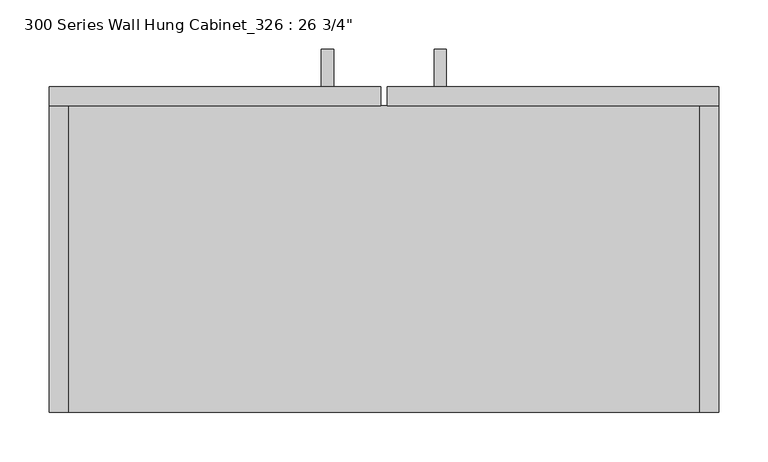
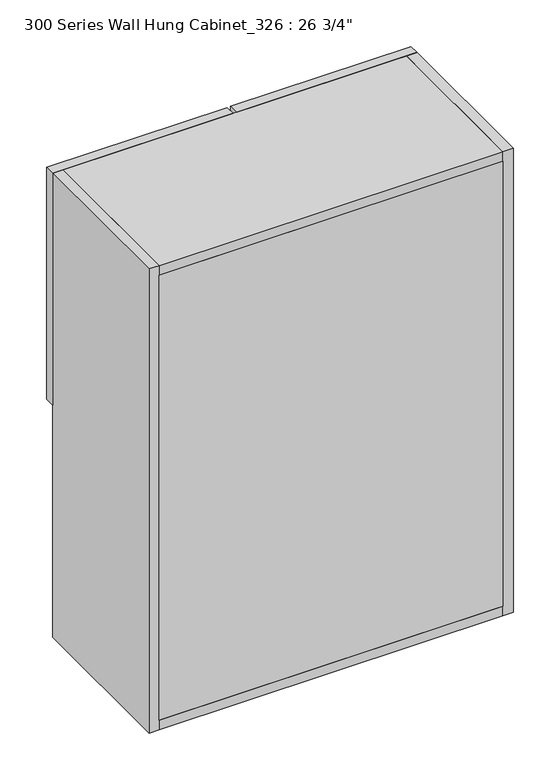
"""IFC4 building model written with IfcOpenShell, lengths in millimetres: furniture geometry."""

from ifc_helpers import new_model, si_unit, frame, origin, place, context, project, spatial, polyline, outline, extrude, source, transform, mapped, element, save


def furniture_b195cdbb(model_context):
    return source(origin(), model_context, "Body", "SweptSolid", [
        extrude(outline(polyline([(406.4, 1809.7425373), (406.4, 1822.4121874), (444.4810937, 1822.4121874), (444.4810937, 1727.2), (406.4, 1727.2), (406.4, 1739.8696501), (431.8114436, 1739.8696501), (431.8114436, 1809.7425373), (406.4, 1809.7425373)])), frame((50.8, 0.0, 0.0), z_axis=(1.0, 0.0, 0.0), x_axis=(0.0, 1.0, 0.0)), (0.0, 0.0, 1.0), 12.4065288),
        extrude(outline(polyline([(406.4, 1809.7425373), (406.4, 1822.4121874), (444.4810937, 1822.4121874), (444.4810937, 1727.2), (406.4, 1727.2), (406.4, 1739.8696501), (431.8114436, 1739.8696501), (431.8114436, 1809.7425373), (406.4, 1809.7425373)])), frame((-63.5, 0.0, 0.0), z_axis=(1.0, 0.0, 0.0), x_axis=(0.0, 1.0, 0.0)), (0.0, 0.0, 1.0), 12.4065288),
        extrude(outline(polyline([(320.675, 387.35), (320.675, 95.25), (-320.675, 95.25), (-320.675, 387.35), (320.675, 387.35)])), frame((0.0, 0.0, 1676.4), z_axis=(0.0, 0.0, 1.0), x_axis=(1.0, 0.0, 0.0)), (0.0, 0.0, 1.0), 19.05),
        extrude(outline(polyline([(320.675, 76.2), (-320.675, 76.2), (-320.675, 95.25), (320.675, 95.25), (320.675, 76.2)])), frame((0.0, 0.0, 1238.25), z_axis=(0.0, 0.0, 1.0), x_axis=(1.0, 0.0, 0.0)), (0.0, 0.0, 1.0), 876.3),
        extrude(outline(polyline([(-3.175, 387.35), (-339.725, 387.35), (-339.725, 406.4), (-3.175, 406.4), (-3.175, 387.35)])), frame((0.0, 0.0, 1676.4), z_axis=(0.0, 0.0, 1.0), x_axis=(1.0, 0.0, 0.0)), (0.0, 0.0, 1.0), 457.2),
        extrude(outline(polyline([(339.725, 387.35), (3.175, 387.35), (3.175, 406.4), (339.725, 406.4), (339.725, 387.35)])), frame((0.0, 0.0, 1676.4), z_axis=(0.0, 0.0, 1.0), x_axis=(1.0, 0.0, 0.0)), (0.0, 0.0, 1.0), 457.2),
        extrude(outline(polyline([(-339.725, 76.2), (-339.725, 387.35), (-320.675, 387.35), (-320.675, 76.2), (-339.725, 76.2)])), frame((0.0, 0.0, 1219.2), z_axis=(0.0, 0.0, 1.0), x_axis=(1.0, 0.0, 0.0)), (0.0, 0.0, 1.0), 914.4),
        extrude(outline(polyline([(320.675, 76.2), (320.675, 387.35), (339.725, 387.35), (339.725, 76.2), (320.675, 76.2)])), frame((0.0, 0.0, 1219.2), z_axis=(0.0, 0.0, 1.0), x_axis=(1.0, 0.0, 0.0)), (0.0, 0.0, 1.0), 914.4),
        extrude(outline(polyline([(320.675, 387.35), (320.675, 76.2), (-320.675, 76.2), (-320.675, 387.35), (320.675, 387.35)])), frame((0.0, 0.0, 2114.55), z_axis=(0.0, 0.0, 1.0), x_axis=(1.0, 0.0, 0.0)), (0.0, 0.0, 1.0), 19.05),
        extrude(outline(polyline([(320.675, 387.35), (320.675, 76.2), (-320.675, 76.2), (-320.675, 387.35), (320.675, 387.35)])), frame((0.0, 0.0, 1219.2), z_axis=(0.0, 0.0, 1.0), x_axis=(1.0, 0.0, 0.0)), (0.0, 0.0, 1.0), 19.05),
    ])


if __name__ == "__main__":
    model = new_model("IFC4")
    model_context = context("Model", 3, world=origin())
    ifc_project = project(units=[si_unit("LENGTHUNIT", "METRE", prefix="MILLI")], contexts=[model_context])
    site = spatial("IfcSite", under=ifc_project)
    building = spatial("IfcBuilding", under=site)
    placement = place(None, origin())
    furniture_shape = furniture_b195cdbb(model_context)
    element("IfcFurniture", 1, ObjectType="300 Series Wall Hung Cabinet_326 : 26 3/4\"", at=placement, inside=building, context=model_context, shape_type="MappedRepresentation", body=[
        mapped(furniture_shape, transform((0.0, 0.0, 0.0), x_axis=(1.0, 0.0, 0.0), y_axis=(0.0, 1.0, 0.0), z_axis=(0.0, 0.0, 1.0))),
    ])
    save(model, "model.ifc")

# Revit data of these elements
# Type "300 Series Wall Hung Cabinet_326 : 26 3/4\""
#   URL = "www.wicnet.org/manual_sections.asp"
#   Model = "326"
#   Manufacturer = "Woodwork Institute"
#   Content Creator URL = "www.AECcontent.com"
#   Content Creator = "AECcontent"
#   Description = "Wall Hung Cabinet"
#   Assembly Code = "E2010200"
#   Width = 2' - 2 3/4"
#   Top of Cabinet = 7' - 0"
#   Height = 3' - 0"
#   Depth = 1' - 1"
#   Top Panel Material = Cabinet
#   Side Panel Material = Cabinet
#   Shelf Panel Material = Cabinet
#   Back Panel Material = Cabinet
#   Door Panel Material = Cabinet
# Element 1 (IfcFurniture, "300 Series Wall Hung Cabinet_326 : 26 3/4\"")
#   Materials on its faces: "Cabinet", "Default metal"
# Materials
#   "Cabinet": class "Wood", colour RGB 189 170 130, transparency 0, Cost = 0
#   "Default metal": class "Unassigned", colour RGB 204 204 204, transparency 0
